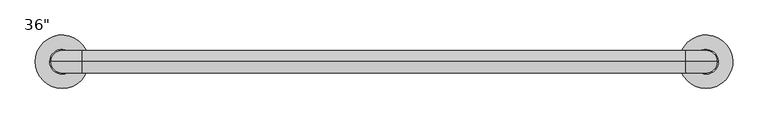
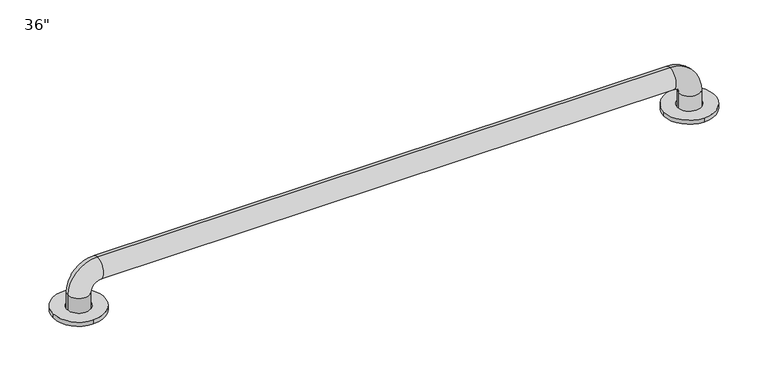
"""IFC4 building model written with IfcOpenShell, lengths in millimetres: proxy geometry."""

import ifcopenshell
import ifcopenshell.guid

model = None  # the IFC model being written
_history = None  # IfcOwnerHistory: only IFC2X3 demands one
_inside = {}  # id of a spatial element -> (the spatial element, [elements in it])
_under = {}  # id of a project, library or spatial element -> (it, [spatial elements below it])
_declared = {}  # id of a project -> (the project, [libraries it declares])
_typed = {}  # id of a type object -> (the type object, [elements of that type])
_made_of = {}  # id of a material, layer set ... -> (it, [elements and type objects made of it])


def new_model(schema):
    """Start an empty IFC model of exactly this schema.

    Asked for "IFC4X3", IfcOpenShell would pick the latest addendum, in which some entities
    have other attributes; the version numbers below select the first issue.
    IFC2X3 requires an IfcOwnerHistory on every rooted entity: one is made here for all.
    """
    global model, _history
    if schema == "IFC4X3":
        model = ifcopenshell.file(schema_version=(4, 3, 0, 0))
    else:
        model = ifcopenshell.file(schema=schema)
    _inside.clear()
    _under.clear()
    _declared.clear()
    _typed.clear()
    _made_of.clear()
    _history = None
    if model.schema == "IFC2X3":
        org = make("IfcOrganization", Name="unknown")
        user = make(
            "IfcPersonAndOrganization",
            ThePerson=make("IfcPerson", FamilyName="unknown"),
            TheOrganization=org,
        )
        app = make(
            "IfcApplication",
            ApplicationDeveloper=org,
            Version="unknown",
            ApplicationFullName="unknown",
            ApplicationIdentifier="unknown",
        )
        _history = make(
            "IfcOwnerHistory",
            OwningUser=user,
            OwningApplication=app,
            ChangeAction="ADDED",
            CreationDate=0,
        )
    return model


def make(cls, **values):
    """One entity of the class cls with the attributes given. An attribute that is None is left unset."""
    return model.create_entity(
        cls, **{name: value for name, value in values.items() if value is not None}
    )


def rooted(cls, **values):
    """An entity with a GlobalId (a new one), such as an element, a storey or a relation."""
    return make(cls, GlobalId=ifcopenshell.guid.new(), OwnerHistory=_history, **values)


def si_unit(unit_type, name, prefix=None):
    """IfcSIUnit, for example si_unit("LENGTHUNIT", "METRE", prefix="MILLI")."""
    return make("IfcSIUnit", UnitType=unit_type, Prefix=prefix, Name=name)


def assignment(units):
    """IfcUnitAssignment: the units of a project."""
    return None if units is None else make("IfcUnitAssignment", Units=units)


def point(xyz):
    """IfcCartesianPoint."""
    return None if xyz is None else make("IfcCartesianPoint", Coordinates=xyz)


def direction(xyz):
    """IfcDirection."""
    return None if xyz is None else make("IfcDirection", DirectionRatios=xyz)


def frame(location, z_axis=None, x_axis=None):
    """IfcAxis2Placement3D, a coordinate frame: its origin and axes. An axis left out is left unset."""
    return make(
        "IfcAxis2Placement3D",
        Location=point(location),
        Axis=direction(z_axis),
        RefDirection=direction(x_axis),
    )


def frame_2d(location, x_axis=None):
    """IfcAxis2Placement2D, a coordinate frame in the plane: its origin and x axis."""
    return make(
        "IfcAxis2Placement2D", Location=point(location), RefDirection=direction(x_axis)
    )


def origin():
    """The frame at (0, 0, 0) with its axes left unset."""
    return frame((0.0, 0.0, 0.0))


def origin_with_axes():
    """The frame at (0, 0, 0) with the z axis (0, 0, 1) and the x axis (1, 0, 0) written out."""
    return frame((0.0, 0.0, 0.0), z_axis=(0.0, 0.0, 1.0), x_axis=(1.0, 0.0, 0.0))


def origin_2d():
    """The frame at (0, 0) in the plane with its x axis left unset."""
    return frame_2d((0.0, 0.0))


def place(relative_to, where):
    """IfcLocalPlacement: puts the frame where relative to a parent placement (None: the world)."""
    return make(
        "IfcLocalPlacement", PlacementRelTo=relative_to, RelativePlacement=where
    )


def context(
    kind, dimensions, precision=None, world=None, true_north=None, identifier=None
):
    """IfcGeometricRepresentationContext, for example the 3D "Model" context."""
    return make(
        "IfcGeometricRepresentationContext",
        ContextIdentifier=identifier,
        ContextType=kind,
        CoordinateSpaceDimension=dimensions,
        Precision=precision,
        WorldCoordinateSystem=world,
        TrueNorth=true_north,
    )


def project(units=None, contexts=None):
    """IfcProject with its units and contexts."""
    return rooted(
        "IfcProject",
        Name="project",
        RepresentationContexts=contexts,
        UnitsInContext=assignment(units),
    )


def spatial(cls, under=None, at=None, **own):
    """A site, building, storey or space (cls), placed at a placement, below another one or the project."""
    s = rooted(cls, ObjectPlacement=at, **own)
    if under is not None:
        _under.setdefault(under.id(), (under, []))[1].append(s)
    return s


def circle_curve(where, radius):
    """IfcCircle in the frame where."""
    return make("IfcCircle", Position=where, Radius=radius)


def ellipse_curve(where, semi_axis1, semi_axis2):
    """IfcEllipse in the frame where."""
    return make(
        "IfcEllipse", Position=where, SemiAxis1=semi_axis1, SemiAxis2=semi_axis2
    )


def trimmed(basis, trim1, trim2, sense, master):
    """IfcTrimmedCurve: the piece of a basis curve between two trims."""
    return make(
        "IfcTrimmedCurve",
        BasisCurve=basis,
        Trim1=trim1,
        Trim2=trim2,
        SenseAgreement=sense,
        MasterRepresentation=master,
    )


def segment(curve, same_sense, transition):
    """IfcCompositeCurveSegment."""
    return make(
        "IfcCompositeCurveSegment",
        Transition=transition,
        SameSense=same_sense,
        ParentCurve=curve,
    )


def composite_curve(segments, self_intersect=None):
    """IfcCompositeCurve: segments joined end to end."""
    return make("IfcCompositeCurve", Segments=segments, SelfIntersect=self_intersect)


def outline(outer, holes=None, kind="AREA"):
    """IfcArbitraryClosedProfileDef: a profile drawn as a closed curve; with holes, ...WithVoids."""
    if holes is None:
        return make("IfcArbitraryClosedProfileDef", ProfileType=kind, OuterCurve=outer)
    return make(
        "IfcArbitraryProfileDefWithVoids",
        ProfileType=kind,
        OuterCurve=outer,
        InnerCurves=holes,
    )


def extrude(swept, where, along, depth):
    """IfcExtrudedAreaSolid: the profile swept, set in the frame where, extruded along a direction by depth."""
    return make(
        "IfcExtrudedAreaSolid",
        SweptArea=swept,
        Position=where,
        ExtrudedDirection=direction(along),
        Depth=depth,
    )


def shape(context_of_items, identifier, shape_type, items):
    """IfcShapeRepresentation: the items that make up one representation, for example the "Body"."""
    return make(
        "IfcShapeRepresentation",
        ContextOfItems=context_of_items,
        RepresentationIdentifier=identifier,
        RepresentationType=shape_type,
        Items=items,
    )


def source(mapping_origin, context_of_items, identifier, shape_type, items):
    """IfcRepresentationMap: a shape defined once, which mapped items show again and again."""
    return make(
        "IfcRepresentationMap",
        MappingOrigin=mapping_origin,
        MappedRepresentation=shape(context_of_items, identifier, shape_type, items),
    )


def transform(
    local_origin,
    x_axis=None,
    y_axis=None,
    z_axis=None,
    scale=None,
    scale2=None,
    scale3=None,
    uniform=True,
):
    """IfcCartesianTransformationOperator3D, or its non-uniform kind. x_axis, y_axis, z_axis: its Axis1, 2, 3."""
    if uniform:
        return make(
            "IfcCartesianTransformationOperator3D",
            Axis1=direction(x_axis),
            Axis2=direction(y_axis),
            LocalOrigin=point(local_origin),
            Scale=scale,
            Axis3=direction(z_axis),
        )
    return make(
        "IfcCartesianTransformationOperator3DnonUniform",
        Axis1=direction(x_axis),
        Axis2=direction(y_axis),
        LocalOrigin=point(local_origin),
        Scale=scale,
        Axis3=direction(z_axis),
        Scale2=scale2,
        Scale3=scale3,
    )


def mapped(mapping_source, mapping_target):
    """IfcMappedItem: shows the shape of a source again, moved by a transform."""
    return make(
        "IfcMappedItem", MappingSource=mapping_source, MappingTarget=mapping_target
    )


def made_of(thing, what):
    """Note that an element or type object is made of a material, layer set ...; save() writes the relation."""
    if what is not None:
        _made_of.setdefault(what.id(), (what, []))[1].append(thing)
    return thing


def element(
    cls,
    number,
    at=None,
    inside=None,
    cuts=None,
    type_object=None,
    material=None,
    context=None,
    identifier="Body",
    shape_type=None,
    held_by="IfcProductDefinitionShape",
    body=None,
    shapes=None,
    **own,
):
    """One element of the class cls, such as IfcWall. Its Tag is "e" and its number.

    at: its placement. inside: the storey or other place that contains it. cuts: it is an
    opening in that element (IfcRelVoidsElement). A single representation is given by context,
    identifier, shape_type and body (its items); several are given by shapes. held_by: the class
    of the entity that holds the representations. save() writes the other relations.
    """
    e = rooted(cls, Tag="e%d" % number, ObjectPlacement=at, **own)
    if body is not None:
        shapes = [shape(context, identifier, shape_type, body)]
    if shapes is not None:
        e.Representation = make(held_by, Representations=shapes)
    if inside is not None:
        _inside.setdefault(inside.id(), (inside, []))[1].append(e)
    if cuts is not None:
        rooted(
            "IfcRelVoidsElement", RelatingBuildingElement=cuts, RelatedOpeningElement=e
        )
    if type_object is not None:
        _typed.setdefault(type_object.id(), (type_object, []))[1].append(e)
    return made_of(e, material)


def aggregate(whole, parts):
    """IfcRelAggregates: a whole, such as a stair, and the parts it consists of."""
    return rooted("IfcRelAggregates", RelatingObject=whole, RelatedObjects=parts)


def save(model, path):
    """Write the relations noted so far, then the file.

    IfcRelAggregates (storeys below a building ...), IfcRelContainedInSpatialStructure (elements
    in a storey), IfcRelDefinesByType, IfcRelAssociatesMaterial and IfcRelDeclares: one each for
    every whole, place, type object, material and project.
    """
    for whole, parts in _under.values():
        aggregate(whole, parts)
    for where, things in _inside.values():
        rooted(
            "IfcRelContainedInSpatialStructure",
            RelatedElements=things,
            RelatingStructure=where,
        )
    for kind, things in _typed.values():
        rooted("IfcRelDefinesByType", RelatedObjects=things, RelatingType=kind)
    for what, things in _made_of.values():
        rooted("IfcRelAssociatesMaterial", RelatedObjects=things, RelatingMaterial=what)
    for by, libraries in _declared.values():
        rooted("IfcRelDeclares", RelatingContext=by, RelatedDefinitions=libraries)
    model.write(path)


def plane_surface(at):
    """IfcPlane: the flat surface through the origin of the frame at, square to its z axis."""
    return make("IfcPlane", Position=at)


def cylinder_surface(at, radius):
    """IfcCylindricalSurface: all points at the distance radius from the z axis of the frame at."""
    return make("IfcCylindricalSurface", Position=at, Radius=radius)


def revolved_surface(curve, axis_point, axis_direction):
    """IfcSurfaceOfRevolution: the curve turned about the line through axis_point along axis_direction."""
    return make(
        "IfcSurfaceOfRevolution",
        SweptCurve=make("IfcArbitraryOpenProfileDef", ProfileType="CURVE", Curve=curve),
        AxisPosition=make("IfcAxis1Placement", Location=point(axis_point), Axis=direction(axis_direction)),
    )


def advanced_brep(points, edges, surfaces, faces):
    """IfcAdvancedBrep: a solid bounded by faces that lie on surfaces and meet in shared edges.

    An edge is (start, end): straight between two places in points (the first is 0);
    or (start, end, curve); or (start, end, curve, False) where it runs against its curve.
    A face is (place in surfaces, loops), or (place, loops, False) where it looks against
    its surface's normal. A loop lists edges by number (the first is 1), with a minus sign
    where the edge is run from its end to its start. The first loop is the outer one.
    """
    corners = [point(p) for p in points]
    vertices = [make("IfcVertexPoint", VertexGeometry=c) for c in corners]
    made = []
    for start, end, *more in edges:
        made.append(
            make(
                "IfcEdgeCurve",
                EdgeStart=vertices[start],
                EdgeEnd=vertices[end],
                EdgeGeometry=more[0] if more else make("IfcPolyline", Points=[corners[start], corners[end]]),
                SameSense=more[1] if len(more) > 1 else True,
            )
        )
    hull = []
    for where, loops, *sense in faces:
        bounds = []
        for j, loop in enumerate(loops):
            ring = [make("IfcOrientedEdge", EdgeElement=made[abs(k) - 1], Orientation=k > 0) for k in loop]
            bounds.append(
                make(
                    "IfcFaceOuterBound" if j == 0 else "IfcFaceBound",
                    Bound=make("IfcEdgeLoop", EdgeList=ring),
                    Orientation=True,
                )
            )
        hull.append(make("IfcAdvancedFace", Bounds=bounds, FaceSurface=surfaces[where], SameSense=sense[0] if sense else True))
    return make("IfcAdvancedBrep", Outer=make("IfcClosedShell", CfsFaces=hull))


def proxy_70f9e0ae(model_context):
    return source(origin(), model_context, "Body", "SolidModel", [
        extrude(outline(composite_curve([segment(trimmed(circle_curve(frame_2d((914.4, 0.0)), 38.1), [point((876.3, 0.0))], [point((914.4, -38.1))], False, "CARTESIAN"), True, "CONTINUOUS"), segment(trimmed(circle_curve(frame_2d((914.4, 0.0)), 38.1), [point((914.4, -38.1))], [point((876.3, 0.0))], False, "CARTESIAN"), True, "CONTINUOUS")], self_intersect=False), holes=[composite_curve([segment(trimmed(circle_curve(frame_2d((914.4, 0.0)), 17.4625), [point((896.9375, 0.0))], [point((914.4, -17.4625))], True, "CARTESIAN"), True, "CONTINUOUS"), segment(trimmed(circle_curve(frame_2d((914.4, 0.0)), 17.4625), [point((914.4, -17.4625))], [point((896.9375, 0.0))], True, "CARTESIAN"), True, "CONTINUOUS")], self_intersect=False)]), origin_with_axes(), (0.0, 0.0, 1.0), 6.35),
        extrude(outline(composite_curve([segment(trimmed(circle_curve(origin_2d(), 38.1), [point((-38.1, 0.0))], [point((0.0, -38.1))], False, "CARTESIAN"), True, "CONTINUOUS"), segment(trimmed(circle_curve(origin_2d(), 38.1), [point((0.0, -38.1))], [point((-38.1, 0.0))], False, "CARTESIAN"), True, "CONTINUOUS")], self_intersect=False), holes=[composite_curve([segment(trimmed(circle_curve(origin_2d(), 17.4625), [point((-17.4625, 0.0))], [point((0.0, -17.4625))], True, "CARTESIAN"), True, "CONTINUOUS"), segment(trimmed(circle_curve(origin_2d(), 17.4625), [point((0.0, -17.4625))], [point((-17.4625, 0.0))], True, "CARTESIAN"), True, "CONTINUOUS")], self_intersect=False)]), origin_with_axes(), (0.0, 0.0, 1.0), 6.35),
        advanced_brep(
        [(930.275, 0.0, 0.0), (898.525, 0.0, 0.0), (930.275, 0.0, 28.575), (898.525, 0.0, 28.575), (885.825, 0.0, 41.275), (885.825, 0.0, 73.025), (28.575, 0.0, 73.025), (28.575, 0.0, 41.275), (15.875, 0.0, 28.575), (-15.875, 0.0, 28.575), (-15.875, 0.0, 0.0), (15.875, 0.0, 0.0)],
        [
            (0, 1, circle_curve(frame((914.4, 0.0, 0.0), z_axis=(0.0, 0.0, -1.0), x_axis=(-1.0, 0.0, 0.0)), 15.875)),
            (1, 0, circle_curve(frame((914.4, 0.0, 0.0), z_axis=(0.0, 0.0, -1.0), x_axis=(-1.0, 0.0, 0.0)), 15.875)),
            (0, 2),
            (2, 3, circle_curve(frame((914.4, 0.0, 28.575), z_axis=(0.0, 0.0, -1.0), x_axis=(-1.0, 0.0, 0.0)), 15.875)),
            (3, 1),
            (3, 2, circle_curve(frame((914.4, 0.0, 28.575), z_axis=(0.0, 0.0, -1.0), x_axis=(-1.0, 0.0, 0.0)), 15.875)),
            (4, 3, circle_curve(frame((885.825, 0.0, 28.575), z_axis=(0.0, 1.0, 0.0), x_axis=(1.0, 0.0, 0.0)), 12.7)),
            (2, 5, circle_curve(frame((885.825, 0.0, 28.575), z_axis=(0.0, -1.0, 0.0), x_axis=(1.0, 0.0, 0.0)), 44.45)),
            (5, 4, circle_curve(frame((885.825, 0.0, 57.15), z_axis=(1.0, 0.0, 0.0), x_axis=(0.0, 0.0, -1.0)), 15.875)),
            (4, 5, circle_curve(frame((885.825, 0.0, 57.15), z_axis=(1.0, 0.0, 0.0), x_axis=(0.0, 0.0, -1.0)), 15.875)),
            (5, 6),
            (6, 7, circle_curve(frame((28.575, 0.0, 57.15), z_axis=(1.0, 0.0, 0.0), x_axis=(0.0, 0.0, -1.0)), 15.875)),
            (7, 4),
            (7, 6, circle_curve(frame((28.575, 0.0, 57.15), z_axis=(1.0, 0.0, 0.0), x_axis=(0.0, 0.0, -1.0)), 15.875)),
            (8, 7, circle_curve(frame((28.575, 0.0, 28.575), z_axis=(0.0, 1.0, 0.0), x_axis=(0.0, 0.0, 1.0)), 12.7)),
            (6, 9, circle_curve(frame((28.575, 0.0, 28.575), z_axis=(0.0, -1.0, 0.0), x_axis=(0.0, 0.0, 1.0)), 44.45)),
            (9, 8, circle_curve(frame((0.0, 0.0, 28.575), z_axis=(0.0, 0.0, 1.0), x_axis=(1.0, 0.0, 0.0)), 15.875)),
            (8, 9, circle_curve(frame((0.0, 0.0, 28.575), z_axis=(0.0, 0.0, 1.0), x_axis=(1.0, 0.0, 0.0)), 15.875)),
            (10, 11, circle_curve(frame((0.0, 0.0, 0.0), z_axis=(0.0, 0.0, -1.0), x_axis=(1.0, 0.0, 0.0)), 15.875)),
            (11, 10, circle_curve(frame((0.0, 0.0, 0.0), z_axis=(0.0, 0.0, -1.0), x_axis=(1.0, 0.0, 0.0)), 15.875)),
            (9, 10),
            (11, 8),
        ],
        [
            plane_surface(frame((914.4, 0.0, 0.0), z_axis=(0.0, 0.0, -1.0), x_axis=(0.0, -1.0, 0.0))),
            cylinder_surface(frame((914.4, 0.0, 0.0), z_axis=(0.0, 0.0, -1.0), x_axis=(-1.0, 0.0, 0.0)), 15.875),
            revolved_surface(trimmed(ellipse_curve(frame((914.4, 0.0, 28.575), z_axis=(0.0, 0.0, -1.0), x_axis=(-1.0, 0.0, 0.0)), 15.875, 15.875), [point((930.275, 0.0, 28.575))], [point((898.525, 0.0, 28.575))], True, "CARTESIAN"), (885.825, 0.0, 28.575), (0.0, -1.0, 0.0)),
            revolved_surface(trimmed(ellipse_curve(frame((914.4, 0.0, 28.575), z_axis=(0.0, 0.0, -1.0), x_axis=(-1.0, 0.0, 0.0)), 15.875, 15.875), [point((898.525, 0.0, 28.575))], [point((930.275, 0.0, 28.575))], True, "CARTESIAN"), (885.825, 0.0, 28.575), (0.0, -1.0, 0.0)),
            cylinder_surface(frame((885.825, 0.0, 57.15), z_axis=(1.0, 0.0, 0.0), x_axis=(0.0, 0.0, -1.0)), 15.875),
            revolved_surface(trimmed(ellipse_curve(frame((28.575, 0.0, 57.15), z_axis=(1.0, 0.0, 0.0), x_axis=(0.0, 0.0, -1.0)), 15.875, 15.875), [point((28.575, 0.0, 73.025))], [point((28.575, 0.0, 41.275))], True, "CARTESIAN"), (28.575, 0.0, 28.575), (0.0, -1.0, 0.0)),
            revolved_surface(trimmed(ellipse_curve(frame((28.575, 0.0, 57.15), z_axis=(1.0, 0.0, 0.0), x_axis=(0.0, 0.0, -1.0)), 15.875, 15.875), [point((28.575, 0.0, 41.275))], [point((28.575, 0.0, 73.025))], True, "CARTESIAN"), (28.575, 0.0, 28.575), (0.0, -1.0, 0.0)),
            plane_surface(frame((0.0, 0.0, 0.0), z_axis=(0.0, 0.0, -1.0), x_axis=(0.0, -1.0, 0.0))),
            cylinder_surface(frame((0.0, 0.0, 28.575), z_axis=(0.0, 0.0, 1.0), x_axis=(1.0, 0.0, 0.0)), 15.875),
        ],
        [
            (0, [[1, 2]]),
            (1, [[-1, 3, 4, 5]]),
            (1, [[-2, -5, 6, -3]]),
            (2, [[7, -4, 8, 9]]),
            (3, [[-8, -6, -7, 10]]),
            (4, [[-9, 11, 12, 13]]),
            (4, [[-10, -13, 14, -11]]),
            (5, [[15, -12, 16, 17]]),
            (6, [[-16, -14, -15, 18]]),
            (7, [[19, 20]]),
            (8, [[-17, 21, -20, 22]]),
            (8, [[-18, -22, -19, -21]]),
        ],
    ),
    ])


if __name__ == "__main__":
    model = new_model("IFC4")
    model_context = context("Model", 3, world=origin())
    ifc_project = project(units=[si_unit("LENGTHUNIT", "METRE", prefix="MILLI")], contexts=[model_context])
    site = spatial("IfcSite", under=ifc_project)
    building = spatial("IfcBuilding", under=site)
    placement = place(None, origin())
    proxy_shape = proxy_70f9e0ae(model_context)
    element("IfcBuildingElementProxy", 1, Name="Seqm-Grab Bar : 36\"", ObjectType="Seqm-Grab Bar : 36\"", at=placement, inside=building, context=model_context, shape_type="MappedRepresentation", body=[
        mapped(proxy_shape, transform((0.0, 0.0, 0.0), x_axis=(1.0, 0.0, 0.0), y_axis=(0.0, 1.0, 0.0), z_axis=(0.0, 0.0, 1.0))),
    ])
    save(model, "model.ifc")

# Revit data of these elements
# Type "Seqm-Grab Bar : 36\""
#   Spec Number = "10 28 00"
#   Spec Description = "36\" GRAB BAR"
#   Length = 3' - 0"
#   Default Elevation = 4' - 0"
#   Grab Bar Material = GRAB BARS - AT ADA RESTROOMS ONLY
# Element 1 (IfcBuildingElementProxy, "Seqm-Grab Bar : 36\"")
#   Materials on its faces: "GRAB BARS - AT ADA RESTROOMS ONLY"
# Materials
#   "GRAB BARS - AT ADA RESTROOMS ONLY": class "Generic", colour RGB 120 120 120, transparency 0, Cost = 0
